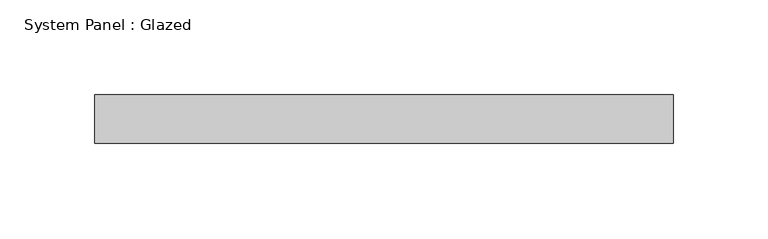
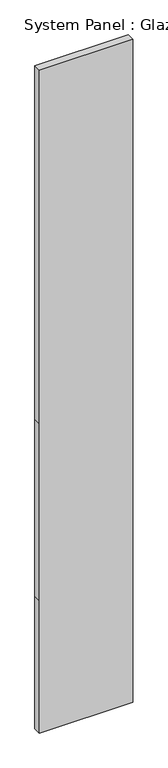
"""IFC4 building model written with IfcOpenShell, lengths in millimetres: plate geometry, System Panel : Glazed."""

import ifcopenshell
import ifcopenshell.guid

model = None  # the IFC model being written
_history = None  # IfcOwnerHistory: only IFC2X3 demands one
_inside = {}  # id of a spatial element -> (the spatial element, [elements in it])
_under = {}  # id of a project, library or spatial element -> (it, [spatial elements below it])
_declared = {}  # id of a project -> (the project, [libraries it declares])
_typed = {}  # id of a type object -> (the type object, [elements of that type])
_made_of = {}  # id of a material, layer set ... -> (it, [elements and type objects made of it])


def new_model(schema):
    """Start an empty IFC model of exactly this schema.

    Asked for "IFC4X3", IfcOpenShell would pick the latest addendum, in which some entities
    have other attributes; the version numbers below select the first issue.
    IFC2X3 requires an IfcOwnerHistory on every rooted entity: one is made here for all.
    """
    global model, _history
    if schema == "IFC4X3":
        model = ifcopenshell.file(schema_version=(4, 3, 0, 0))
    else:
        model = ifcopenshell.file(schema=schema)
    _inside.clear()
    _under.clear()
    _declared.clear()
    _typed.clear()
    _made_of.clear()
    _history = None
    if model.schema == "IFC2X3":
        org = make("IfcOrganization", Name="unknown")
        user = make(
            "IfcPersonAndOrganization",
            ThePerson=make("IfcPerson", FamilyName="unknown"),
            TheOrganization=org,
        )
        app = make(
            "IfcApplication",
            ApplicationDeveloper=org,
            Version="unknown",
            ApplicationFullName="unknown",
            ApplicationIdentifier="unknown",
        )
        _history = make(
            "IfcOwnerHistory",
            OwningUser=user,
            OwningApplication=app,
            ChangeAction="ADDED",
            CreationDate=0,
        )
    return model


def make(cls, **values):
    """One entity of the class cls with the attributes given. An attribute that is None is left unset."""
    return model.create_entity(
        cls, **{name: value for name, value in values.items() if value is not None}
    )


def rooted(cls, **values):
    """An entity with a GlobalId (a new one), such as an element, a storey or a relation."""
    return make(cls, GlobalId=ifcopenshell.guid.new(), OwnerHistory=_history, **values)


def si_unit(unit_type, name, prefix=None):
    """IfcSIUnit, for example si_unit("LENGTHUNIT", "METRE", prefix="MILLI")."""
    return make("IfcSIUnit", UnitType=unit_type, Prefix=prefix, Name=name)


def assignment(units):
    """IfcUnitAssignment: the units of a project."""
    return None if units is None else make("IfcUnitAssignment", Units=units)


def point(xyz):
    """IfcCartesianPoint."""
    return None if xyz is None else make("IfcCartesianPoint", Coordinates=xyz)


def direction(xyz):
    """IfcDirection."""
    return None if xyz is None else make("IfcDirection", DirectionRatios=xyz)


def frame(location, z_axis=None, x_axis=None):
    """IfcAxis2Placement3D, a coordinate frame: its origin and axes. An axis left out is left unset."""
    return make(
        "IfcAxis2Placement3D",
        Location=point(location),
        Axis=direction(z_axis),
        RefDirection=direction(x_axis),
    )


def origin():
    """The frame at (0, 0, 0) with its axes left unset."""
    return frame((0.0, 0.0, 0.0))


def place(relative_to, where):
    """IfcLocalPlacement: puts the frame where relative to a parent placement (None: the world)."""
    return make(
        "IfcLocalPlacement", PlacementRelTo=relative_to, RelativePlacement=where
    )


def context(
    kind, dimensions, precision=None, world=None, true_north=None, identifier=None
):
    """IfcGeometricRepresentationContext, for example the 3D "Model" context."""
    return make(
        "IfcGeometricRepresentationContext",
        ContextIdentifier=identifier,
        ContextType=kind,
        CoordinateSpaceDimension=dimensions,
        Precision=precision,
        WorldCoordinateSystem=world,
        TrueNorth=true_north,
    )


def project(units=None, contexts=None):
    """IfcProject with its units and contexts."""
    return rooted(
        "IfcProject",
        Name="project",
        RepresentationContexts=contexts,
        UnitsInContext=assignment(units),
    )


def spatial(cls, under=None, at=None, **own):
    """A site, building, storey or space (cls), placed at a placement, below another one or the project."""
    s = rooted(cls, ObjectPlacement=at, **own)
    if under is not None:
        _under.setdefault(under.id(), (under, []))[1].append(s)
    return s


def polyline(points):
    """IfcPolyline through the points."""
    return make("IfcPolyline", Points=[point(p) for p in points])


def outline(outer, holes=None, kind="AREA"):
    """IfcArbitraryClosedProfileDef: a profile drawn as a closed curve; with holes, ...WithVoids."""
    if holes is None:
        return make("IfcArbitraryClosedProfileDef", ProfileType=kind, OuterCurve=outer)
    return make(
        "IfcArbitraryProfileDefWithVoids",
        ProfileType=kind,
        OuterCurve=outer,
        InnerCurves=holes,
    )


def extrude(swept, where, along, depth):
    """IfcExtrudedAreaSolid: the profile swept, set in the frame where, extruded along a direction by depth."""
    return make(
        "IfcExtrudedAreaSolid",
        SweptArea=swept,
        Position=where,
        ExtrudedDirection=direction(along),
        Depth=depth,
    )


def shape(context_of_items, identifier, shape_type, items):
    """IfcShapeRepresentation: the items that make up one representation, for example the "Body"."""
    return make(
        "IfcShapeRepresentation",
        ContextOfItems=context_of_items,
        RepresentationIdentifier=identifier,
        RepresentationType=shape_type,
        Items=items,
    )


def source(mapping_origin, context_of_items, identifier, shape_type, items):
    """IfcRepresentationMap: a shape defined once, which mapped items show again and again."""
    return make(
        "IfcRepresentationMap",
        MappingOrigin=mapping_origin,
        MappedRepresentation=shape(context_of_items, identifier, shape_type, items),
    )


def transform(
    local_origin,
    x_axis=None,
    y_axis=None,
    z_axis=None,
    scale=None,
    scale2=None,
    scale3=None,
    uniform=True,
):
    """IfcCartesianTransformationOperator3D, or its non-uniform kind. x_axis, y_axis, z_axis: its Axis1, 2, 3."""
    if uniform:
        return make(
            "IfcCartesianTransformationOperator3D",
            Axis1=direction(x_axis),
            Axis2=direction(y_axis),
            LocalOrigin=point(local_origin),
            Scale=scale,
            Axis3=direction(z_axis),
        )
    return make(
        "IfcCartesianTransformationOperator3DnonUniform",
        Axis1=direction(x_axis),
        Axis2=direction(y_axis),
        LocalOrigin=point(local_origin),
        Scale=scale,
        Axis3=direction(z_axis),
        Scale2=scale2,
        Scale3=scale3,
    )


def mapped(mapping_source, mapping_target):
    """IfcMappedItem: shows the shape of a source again, moved by a transform."""
    return make(
        "IfcMappedItem", MappingSource=mapping_source, MappingTarget=mapping_target
    )


def made_of(thing, what):
    """Note that an element or type object is made of a material, layer set ...; save() writes the relation."""
    if what is not None:
        _made_of.setdefault(what.id(), (what, []))[1].append(thing)
    return thing


def element(
    cls,
    number,
    at=None,
    inside=None,
    cuts=None,
    type_object=None,
    material=None,
    context=None,
    identifier="Body",
    shape_type=None,
    held_by="IfcProductDefinitionShape",
    body=None,
    shapes=None,
    **own,
):
    """One element of the class cls, such as IfcWall. Its Tag is "e" and its number.

    at: its placement. inside: the storey or other place that contains it. cuts: it is an
    opening in that element (IfcRelVoidsElement). A single representation is given by context,
    identifier, shape_type and body (its items); several are given by shapes. held_by: the class
    of the entity that holds the representations. save() writes the other relations.
    """
    e = rooted(cls, Tag="e%d" % number, ObjectPlacement=at, **own)
    if body is not None:
        shapes = [shape(context, identifier, shape_type, body)]
    if shapes is not None:
        e.Representation = make(held_by, Representations=shapes)
    if inside is not None:
        _inside.setdefault(inside.id(), (inside, []))[1].append(e)
    if cuts is not None:
        rooted(
            "IfcRelVoidsElement", RelatingBuildingElement=cuts, RelatedOpeningElement=e
        )
    if type_object is not None:
        _typed.setdefault(type_object.id(), (type_object, []))[1].append(e)
    return made_of(e, material)


def aggregate(whole, parts):
    """IfcRelAggregates: a whole, such as a stair, and the parts it consists of."""
    return rooted("IfcRelAggregates", RelatingObject=whole, RelatedObjects=parts)


def save(model, path):
    """Write the relations noted so far, then the file.

    IfcRelAggregates (storeys below a building ...), IfcRelContainedInSpatialStructure (elements
    in a storey), IfcRelDefinesByType, IfcRelAssociatesMaterial and IfcRelDeclares: one each for
    every whole, place, type object, material and project.
    """
    for whole, parts in _under.values():
        aggregate(whole, parts)
    for where, things in _inside.values():
        rooted(
            "IfcRelContainedInSpatialStructure",
            RelatedElements=things,
            RelatingStructure=where,
        )
    for kind, things in _typed.values():
        rooted("IfcRelDefinesByType", RelatedObjects=things, RelatingType=kind)
    for what, things in _made_of.values():
        rooted("IfcRelAssociatesMaterial", RelatedObjects=things, RelatingMaterial=what)
    for by, libraries in _declared.values():
        rooted("IfcRelDeclares", RelatingContext=by, RelatedDefinitions=libraries)
    model.write(path)


def system_panel_glazed_14f47568(model_context):
    return source(origin(), model_context, "Body", "SweptSolid", [
        extrude(outline(polyline([(0.0, -152.4), (0.0, 152.4), (457.2, 152.4), (1066.8, 152.4), (2286.0, 152.4), (2286.0, -152.4), (1066.8, -152.4), (457.2, -152.4), (0.0, -152.4)])), frame((0.0, -44.45, 0.0), z_axis=(0.0, 1.0, 0.0), x_axis=(0.0, 0.0, 1.0)), (0.0, 0.0, 1.0), 25.4),
    ])


if __name__ == "__main__":
    model = new_model("IFC4")
    model_context = context("Model", 3, world=origin())
    ifc_project = project(units=[si_unit("LENGTHUNIT", "METRE", prefix="MILLI")], contexts=[model_context])
    site = spatial("IfcSite", under=ifc_project)
    building = spatial("IfcBuilding", under=site)
    placement = place(None, origin())
    system_panel_glazed_shape = system_panel_glazed_14f47568(model_context)
    element("IfcPlate", 1, ObjectType="System Panel : Glazed", at=placement, inside=building, context=model_context, shape_type="MappedRepresentation", body=[
        mapped(system_panel_glazed_shape, transform((0.0, 0.0, 0.0), x_axis=(1.0, 0.0, 0.0), y_axis=(0.0, 1.0, 0.0), z_axis=(0.0, 0.0, 1.0))),
    ])
    save(model, "model.ifc")

# Revit data of these elements
# Element 1 (IfcPlate, "System Panel : Glazed")
#   Materials on its faces: "Glass"
# Materials
#   "Glass": class "Glass", colour RGB 0 128 192, transparency 0.75
